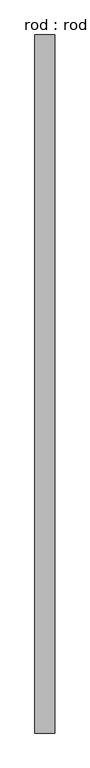
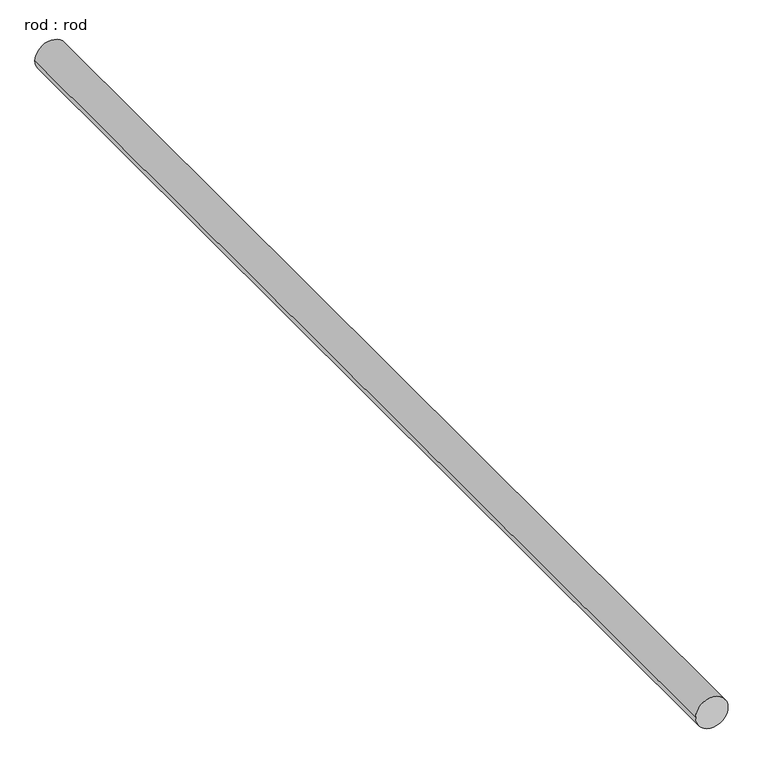
"""IFC4 building model written with IfcOpenShell, lengths in millimetres: proxy geometry, rod : rod."""

from ifc_helpers import new_model, si_unit, point, frame, frame_2d, origin, place, context, project, spatial, circle_curve, trimmed, segment, composite_curve, outline, extrude, source, transform, mapped, element, save


def rod_rod_1aeb8aaf(model_context):
    return source(origin(), model_context, "Body", "SweptSolid", [
        extrude(outline(composite_curve([segment(trimmed(circle_curve(frame_2d((0.0108462, 0.0)), 200.0), [point((0.0108462, 200.0))], [point((0.0108462, -200.0))], False, "CARTESIAN"), True, "CONTINUOUS"), segment(trimmed(circle_curve(frame_2d((0.0108462, 0.0)), 200.0), [point((0.0108462, -200.0))], [point((0.0108462, 200.0))], False, "CARTESIAN"), True, "CONTINUOUS")], self_intersect=False)), frame((0.0, -2992.0928132, 0.0), z_axis=(0.0, 1.0, 0.0), x_axis=(0.0, 0.0, 1.0)), (0.0, 0.0, 1.0), 14169.6428571),
    ])


if __name__ == "__main__":
    model = new_model("IFC4")
    model_context = context("Model", 3, world=origin())
    ifc_project = project(units=[si_unit("LENGTHUNIT", "METRE", prefix="MILLI")], contexts=[model_context])
    site = spatial("IfcSite", under=ifc_project)
    building = spatial("IfcBuilding", under=site)
    placement = place(None, origin())
    rod_rod_shape = rod_rod_1aeb8aaf(model_context)
    element("IfcBuildingElementProxy", 1, Name="rod : rod", ObjectType="rod : rod", at=placement, inside=building, context=model_context, shape_type="MappedRepresentation", body=[
        mapped(rod_rod_shape, transform((0.0, 0.0, 0.0), x_axis=(1.0, 0.0, 0.0), y_axis=(0.0, 1.0, 0.0), z_axis=(0.0, 0.0, 1.0))),
    ])
    save(model, "model.ifc")

# Revit data of these elements
# Type "rod : rod"
#   Default Elevation = 0
